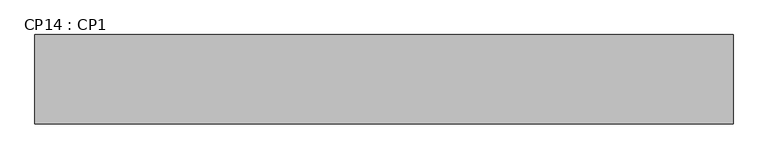
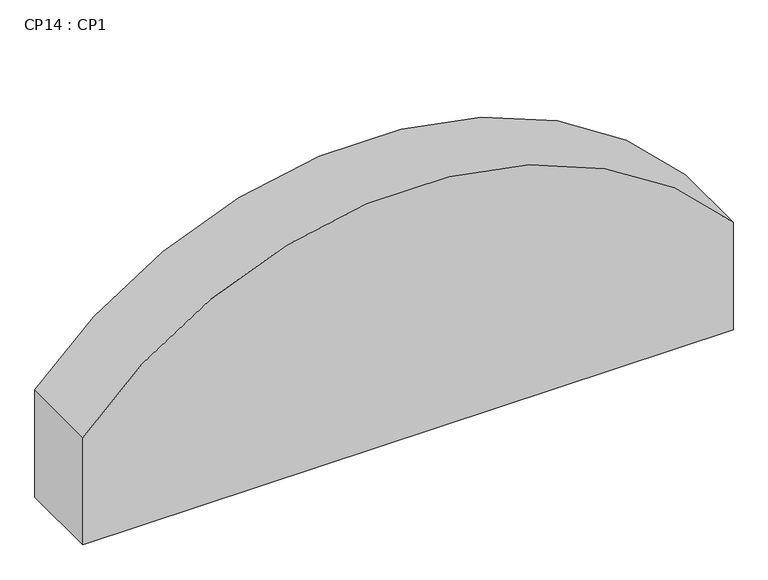
"""IFC4 building model written with IfcOpenShell, lengths in millimetres: beam geometry, CP14 : CP1."""

from ifc_helpers import new_model, si_unit, frame, origin, place, context, project, spatial, circle_curve, source, transform, mapped, element, save
from ifc_brep_helpers import plane_surface, cylinder_surface, advanced_brep


def cp14_cp1_5301f1b9(model_context):
    return source(origin(), model_context, "Body", "AdvancedBrep", [
        advanced_brep(
        [(20143.2245533, 20099.7448193, 13800.0), (20143.2245533, 20099.7448193, 14620.0), (24843.2245539, 20099.7448193, 14620.0), (24843.2245539, 20099.7448193, 13800.0), (24843.2245539, 19499.6999972, 14620.0), (20143.224554, 19499.6999972, 14620.0), (20143.2245533, 19499.6999972, 13800.0), (24843.2245539, 19499.6999972, 13800.0)],
        [
            (0, 1),
            (1, 2, circle_curve(frame((22493.2245539, 20099.7448193, 12608.2612414), z_axis=(0.0, 1.0, 0.0), x_axis=(0.0, 0.0, -1.0)), 3093.4758497)),
            (2, 3),
            (3, 0),
            (4, 5, circle_curve(frame((22493.2245539, 19499.6999972, 12608.2612414), z_axis=(0.0, -1.0, 0.0), x_axis=(0.0, 0.0, -1.0)), 3093.4758497)),
            (5, 6),
            (6, 7),
            (7, 4),
            (6, 0),
            (3, 7),
            (4, 2),
            (1, 5),
        ],
        [
            plane_surface(frame((19993.2245542, 20099.7448193, 13800.0), z_axis=(0.0, 1.0, 0.0), x_axis=(-1.0, 0.0, 0.0))),
            plane_surface(frame((19993.2245542, 19499.6999972, 13800.0), z_axis=(0.0, -1.0, 0.0), x_axis=(1.0, 0.0, 0.0))),
            plane_surface(frame((25143.2245539, 20099.7448193, 13800.0), z_axis=(0.0, 0.0, -1.0), x_axis=(0.0, -1.0, 0.0))),
            cylinder_surface(frame((22493.2245539, 20099.7448193, 12608.2612414), z_axis=(0.0, 1.0, 0.0), x_axis=(0.0, 0.0, -1.0)), 3093.4758497),
            plane_surface(frame((20143.2245533, 18587.0448193, 14620.0), z_axis=(-1.0, 0.0, 0.0), x_axis=(0.0, -1.0, 0.0))),
            plane_surface(frame((24843.2245539, 18587.0448193, 13800.0), z_axis=(1.0, 0.0, 0.0), x_axis=(0.0, -1.0, 0.0))),
        ],
        [
            (0, [[1, 2, 3, 4]]),
            (1, [[5, 6, 7, 8]]),
            (2, [[9, -4, 10, -7]]),
            (3, [[-5, 11, -2, 12]]),
            (4, [[-1, -9, -6, -12]]),
            (5, [[-3, -11, -8, -10]]),
        ],
    ),
    ])


if __name__ == "__main__":
    model = new_model("IFC4")
    model_context = context("Model", 3, world=origin())
    ifc_project = project(units=[si_unit("LENGTHUNIT", "METRE", prefix="MILLI")], contexts=[model_context])
    site = spatial("IfcSite", under=ifc_project)
    building = spatial("IfcBuilding", under=site)
    placement = place(None, origin())
    cp14_cp1_shape = cp14_cp1_5301f1b9(model_context)
    element("IfcBeam", 1, ObjectType="CP14 : CP1", at=placement, inside=building, context=model_context, shape_type="MappedRepresentation", body=[
        mapped(cp14_cp1_shape, transform((0.0, 0.0, 0.0), x_axis=(1.0, 0.0, 0.0), y_axis=(0.0, 1.0, 0.0), z_axis=(0.0, 0.0, 1.0))),
    ])
    save(model, "model.ifc")
